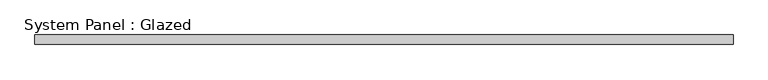
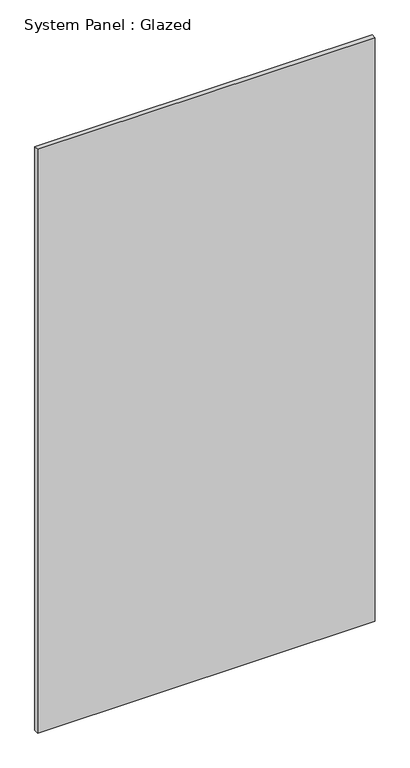
"""IFC4 building model written with IfcOpenShell, lengths in millimetres: plate geometry, System Panel : Glazed."""

from ifc_helpers import new_model, si_unit, origin, origin_with_axes, place, context, project, spatial, polyline, outline, extrude, source, transform, mapped, element, save


def system_panel_glazed_f294eff5(model_context):
    return source(origin(), model_context, "Body", "SweptSolid", [
        extrude(outline(polyline([(922.1913812, 24.5), (-922.1913812, 24.5), (-922.1913812, 49.5), (922.1913812, 49.5), (922.1913812, 24.5)])), origin_with_axes(), (0.0, 0.0, 1.0), 3370.0),
    ])


if __name__ == "__main__":
    model = new_model("IFC4")
    model_context = context("Model", 3, world=origin())
    ifc_project = project(units=[si_unit("LENGTHUNIT", "METRE", prefix="MILLI")], contexts=[model_context])
    site = spatial("IfcSite", under=ifc_project)
    building = spatial("IfcBuilding", under=site)
    placement = place(None, origin())
    system_panel_glazed_shape = system_panel_glazed_f294eff5(model_context)
    element("IfcPlate", 1, ObjectType="System Panel : Glazed", at=placement, inside=building, context=model_context, shape_type="MappedRepresentation", body=[
        mapped(system_panel_glazed_shape, transform((0.0, 0.0, 0.0), x_axis=(1.0, 0.0, 0.0), y_axis=(0.0, 1.0, 0.0), z_axis=(0.0, 0.0, 1.0))),
    ])
    save(model, "model.ifc")

# Revit data of these elements
# Type "System Panel : Glazed"
#   Construction Type Id = "GSP4R"
#   Analytic Construction = "1/8 in Pilkington single glazing"
#   Visual Light Transmittance = 0.9
#   Solar Heat Gain Coefficient = 0.86
#   Heat Transfer Coefficient (U) = 6.7069 W/(m²·K)
#   Define Thermal Properties by = 1
# Element 1 (IfcPlate, "System Panel : Glazed")
#   Materials on its faces: "Glass"
# Materials
#   "Glass": class "Glass", colour RGB 245 245 243, transparency 1, Description = "Soda Lime Glass", Cost = 0
